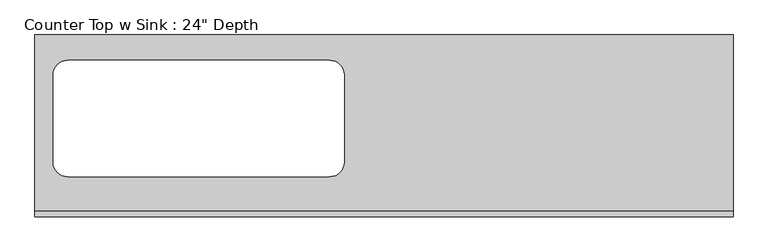
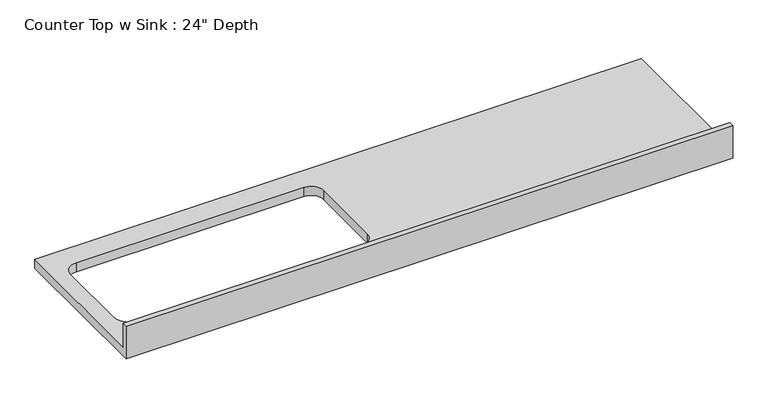
"""IFC4 building model written with IfcOpenShell, lengths in millimetres: furniture geometry."""

from ifc_helpers import new_model, si_unit, frame, origin, place, context, project, spatial, polyline, circle_curve, source, transform, mapped, element, save
from ifc_brep_helpers import plane_surface, revolved_surface, advanced_brep


def furniture_ebdcb837(model_context):
    return source(origin(), model_context, "Body", "AdvancedBrep", [
        advanced_brep(
        [(-1200.4622951, 635.0, 914.4), (-1200.4622951, 19.05, 914.4), (1237.9377049, 19.05, 914.4), (1237.9377049, 635.0, 914.4), (-1086.1622951, 139.7, 914.4), (-1136.9622951, 190.5, 914.4), (-1136.9622951, 495.3, 914.4), (-1086.1622951, 546.1, 914.4), (-171.7622951, 546.1, 914.4), (-120.9622951, 495.3, 914.4), (-120.9622951, 190.5, 914.4), (-171.7622951, 139.7, 914.4), (1237.9377049, 0.0, 876.3), (-1200.4622951, 0.0, 876.3), (-1200.4622951, 635.0, 876.3), (1237.9377049, 635.0, 876.3), (-171.7622951, 139.7, 876.3), (-120.9622951, 190.5, 876.3), (-120.9622951, 495.3, 876.3), (-171.7622951, 546.1, 876.3), (-1086.1622951, 546.1, 876.3), (-1136.9622951, 495.3, 876.3), (-1136.9622951, 190.5, 876.3), (-1086.1622951, 139.7, 876.3), (1237.9377049, 0.0, 1016.0), (-1200.4622951, 0.0, 1016.0), (-1200.4622951, 19.05, 1016.0), (1237.9377049, 19.05, 1016.0)],
        [
            (0, 1),
            (1, 2),
            (2, 3),
            (3, 0),
            (4, 5, circle_curve(frame((-1086.1622951, 190.5, 914.4), z_axis=(0.0, 0.0, -1.0), x_axis=(1.0, 0.0, 0.0)), 50.8)),
            (5, 6),
            (6, 7, circle_curve(frame((-1086.1622951, 495.3, 914.4), z_axis=(0.0, 0.0, -1.0), x_axis=(1.0, 0.0, 0.0)), 50.8)),
            (7, 8),
            (8, 9, circle_curve(frame((-171.7622951, 495.3, 914.4), z_axis=(0.0, 0.0, -1.0), x_axis=(1.0, 0.0, 0.0)), 50.8)),
            (9, 10),
            (10, 11, circle_curve(frame((-171.7622951, 190.5, 914.4), z_axis=(0.0, 0.0, -1.0), x_axis=(1.0, 0.0, 0.0)), 50.8)),
            (11, 4),
            (12, 13),
            (13, 14),
            (14, 15),
            (15, 12),
            (16, 17, circle_curve(frame((-171.7622951, 190.5, 876.3), z_axis=(0.0, 0.0, 1.0), x_axis=(1.0, 0.0, 0.0)), 50.8)),
            (17, 18),
            (18, 19, circle_curve(frame((-171.7622951, 495.3, 876.3), z_axis=(0.0, 0.0, 1.0), x_axis=(1.0, 0.0, 0.0)), 50.8)),
            (19, 20),
            (20, 21, circle_curve(frame((-1086.1622951, 495.3, 876.3), z_axis=(0.0, 0.0, 1.0), x_axis=(1.0, 0.0, 0.0)), 50.8)),
            (21, 22),
            (22, 23, circle_curve(frame((-1086.1622951, 190.5, 876.3), z_axis=(0.0, 0.0, 1.0), x_axis=(1.0, 0.0, 0.0)), 50.8)),
            (23, 16),
            (12, 24),
            (24, 25),
            (25, 13),
            (25, 26),
            (26, 1),
            (0, 14),
            (3, 15),
            (2, 27),
            (27, 24),
            (27, 26),
            (11, 16),
            (23, 4),
            (22, 5),
            (21, 6),
            (20, 7),
            (19, 8),
            (18, 9),
            (17, 10),
        ],
        [
            plane_surface(frame((-1200.4622951, 0.0, 914.4), z_axis=(0.0, 0.0, 1.0), x_axis=(-1.0, 0.0, 0.0))),
            plane_surface(frame((-1200.4622951, 0.0, 876.3), z_axis=(0.0, 0.0, -1.0), x_axis=(1.0, 0.0, 0.0))),
            plane_surface(frame((1237.9377049, 0.0, 914.4), z_axis=(0.0, -1.0, 0.0), x_axis=(0.0, 0.0, -1.0))),
            plane_surface(frame((-1200.4622951, 0.0, 914.4), z_axis=(-1.0, 0.0, 0.0), x_axis=(0.0, 0.0, -1.0))),
            plane_surface(frame((-1200.4622951, 635.0, 914.4), z_axis=(0.0, 1.0, 0.0), x_axis=(0.0, 0.0, -1.0))),
            plane_surface(frame((1237.9377049, 635.0, 914.4), z_axis=(1.0, 0.0, 0.0), x_axis=(0.0, 0.0, -1.0))),
            plane_surface(frame((-1200.4622951, 0.0, 1016.0), z_axis=(0.0, 0.0, 1.0), x_axis=(0.0, 1.0, 0.0))),
            plane_surface(frame((-1200.4622951, 19.05, 1016.0), z_axis=(0.0, 1.0, 0.0), x_axis=(0.0, 0.0, -1.0))),
            plane_surface(frame((-171.7622951, 139.7, 914.4), z_axis=(0.0, 1.0, 0.0), x_axis=(0.0, 0.0, -1.0))),
            revolved_surface(polyline([(-1035.3622951, 190.5, 914.4), (-1035.3622951, 190.5, 876.3)]), (-1086.1622951, 190.5, 876.3), (0.0, 0.0, 1.0)),
            plane_surface(frame((-1136.9622951, 190.5, 914.4), z_axis=(1.0, 0.0, 0.0), x_axis=(0.0, 0.0, -1.0))),
            revolved_surface(polyline([(-1035.3622951, 495.3, 914.4), (-1035.3622951, 495.3, 876.3)]), (-1086.1622951, 495.3, 876.3), (0.0, 0.0, 1.0)),
            plane_surface(frame((-1086.1622951, 546.1, 914.4), z_axis=(0.0, -1.0, 0.0), x_axis=(0.0, 0.0, -1.0))),
            revolved_surface(polyline([(-120.96229509999999, 495.3, 914.4), (-120.96229509999999, 495.3, 876.3)]), (-171.7622951, 495.3, 876.3), (0.0, 0.0, 1.0)),
            plane_surface(frame((-120.9622951, 495.3, 914.4), z_axis=(-1.0, 0.0, 0.0), x_axis=(0.0, 0.0, -1.0))),
            revolved_surface(polyline([(-120.96229509999999, 190.5, 914.4), (-120.96229509999999, 190.5, 876.3)]), (-171.7622951, 190.5, 876.3), (0.0, 0.0, 1.0)),
        ],
        [
            (0, [[1, 2, 3, 4], [5, 6, 7, 8, 9, 10, 11, 12]]),
            (1, [[13, 14, 15, 16], [17, 18, 19, 20, 21, 22, 23, 24]]),
            (2, [[25, 26, 27, -13]]),
            (3, [[-27, 28, 29, -1, 30, -14]]),
            (4, [[31, -15, -30, -4]]),
            (5, [[-31, -3, 32, 33, -25, -16]]),
            (6, [[-26, -33, 34, -28]]),
            (7, [[-32, -2, -29, -34]]),
            (8, [[-12, 35, -24, 36]]),
            (9, [[-23, 37, -5, -36]]),
            (10, [[-22, 38, -6, -37]]),
            (11, [[-21, 39, -7, -38]]),
            (12, [[-20, 40, -8, -39]]),
            (13, [[-19, 41, -9, -40]]),
            (14, [[-18, 42, -10, -41]]),
            (15, [[-11, -42, -17, -35]]),
        ],
    ),
    ])


if __name__ == "__main__":
    model = new_model("IFC4")
    model_context = context("Model", 3, world=origin())
    ifc_project = project(units=[si_unit("LENGTHUNIT", "METRE", prefix="MILLI")], contexts=[model_context])
    site = spatial("IfcSite", under=ifc_project)
    building = spatial("IfcBuilding", under=site)
    placement = place(None, origin())
    furniture_shape = furniture_ebdcb837(model_context)
    element("IfcFurniture", 1, ObjectType="Counter Top w Sink : 24\" Depth", at=placement, inside=building, context=model_context, shape_type="MappedRepresentation", body=[
        mapped(furniture_shape, transform((0.0, 0.0, 0.0), x_axis=(1.0, 0.0, 0.0), y_axis=(0.0, 1.0, 0.0), z_axis=(0.0, 0.0, 1.0))),
    ])
    save(model, "model.ifc")

# Revit data of these elements
# Type "Counter Top w Sink : 24\" Depth"
#   Assembly Code = "C1030400"
#   Counter Thickness = 0' - 1 1/2"
#   Depth = 2' - 1"
#   Height = 3' - 0"
#   Length [instance default] = 8' - 0"
#   Sink Location [instance default] = 2' - 0"
#   Sink Location To Wall [instance default] = 0' - 6"
#   Sink Opening Depth [instance default] = 1' - 3"
#   Sink Opening Width [instance default] = 3' - 3"
#   Counter Top Material = none
#   Default Elevation = 0
# Element 1 (IfcFurniture, "Counter Top w Sink : 24\" Depth")
#   Sink Location = 1' - 10 1/2"
#   Materials on its faces: "Laminate"
# Materials
#   "Laminate": class "Unassigned", colour RGB 247 235 201, transparency 0
